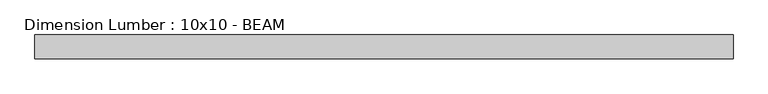
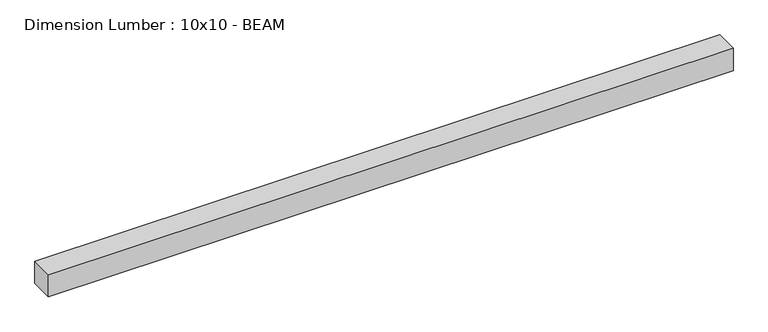
"""IFC4 building model written with IfcOpenShell, lengths in millimetres: beam geometry, Dimension Lumber : 10x10 - BEAM."""

from ifc_helpers import new_model, si_unit, frame, origin, place, context, project, spatial, polyline, outline, extrude, source, transform, mapped, element, save


def dimension_lumber_10x10_beam_780dcf97(model_context):
    return source(origin(), model_context, "Body", "SweptSolid", [
        extrude(outline(polyline([(3429.0, 117.475), (3429.0, -117.475), (-3429.0, -117.475), (-3429.0, 117.475), (3429.0, 117.475)])), frame((0.0, 0.0, -117.475), z_axis=(0.0, 0.0, 1.0), x_axis=(1.0, 0.0, 0.0)), (0.0, 0.0, 1.0), 234.95),
    ])


if __name__ == "__main__":
    model = new_model("IFC4")
    model_context = context("Model", 3, world=origin())
    ifc_project = project(units=[si_unit("LENGTHUNIT", "METRE", prefix="MILLI")], contexts=[model_context])
    site = spatial("IfcSite", under=ifc_project)
    building = spatial("IfcBuilding", under=site)
    placement = place(None, origin())
    dimension_lumber_10x10_beam_shape = dimension_lumber_10x10_beam_780dcf97(model_context)
    element("IfcBeam", 1, ObjectType="Dimension Lumber : 10x10 - BEAM", at=placement, inside=building, context=model_context, shape_type="MappedRepresentation", body=[
        mapped(dimension_lumber_10x10_beam_shape, transform((0.0, 0.0, 0.0), x_axis=(1.0, 0.0, 0.0), y_axis=(0.0, 1.0, 0.0), z_axis=(0.0, 0.0, 1.0))),
    ])
    save(model, "model.ifc")

# Revit data of these elements
# Type "Dimension Lumber : 10x10 - BEAM"
#   Assembly Code = "B10"
#   A = 0.0755556 SF
#   Length [instance default] = 5' - 0"
#   b = 0' - 9 1/4"
#   d = 0' - 9 1/4"
#   Structural Material = (4) CHARRED SISTERED 2X10s AT BEAM
# Element 1 (IfcBeam, "Dimension Lumber : 10x10 - BEAM")
#   Materials on its faces: "(4) CHARRED SISTERED 2X10s AT BEAM"
# Materials
#   "(4) CHARRED SISTERED 2X10s AT BEAM": class "Wood", colour RGB 144 144 144, transparency 0, Description = "Pinus Echinata", Cost = 0
